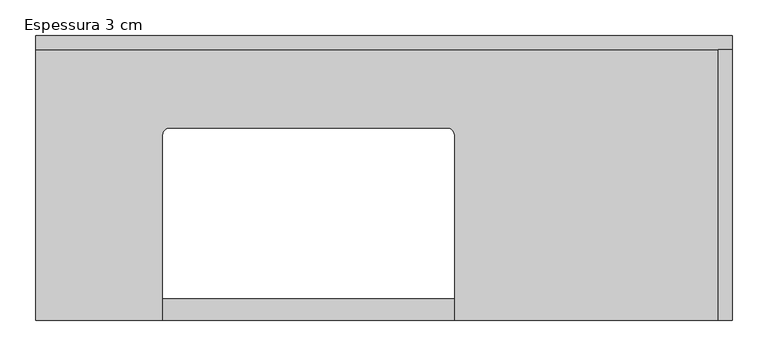
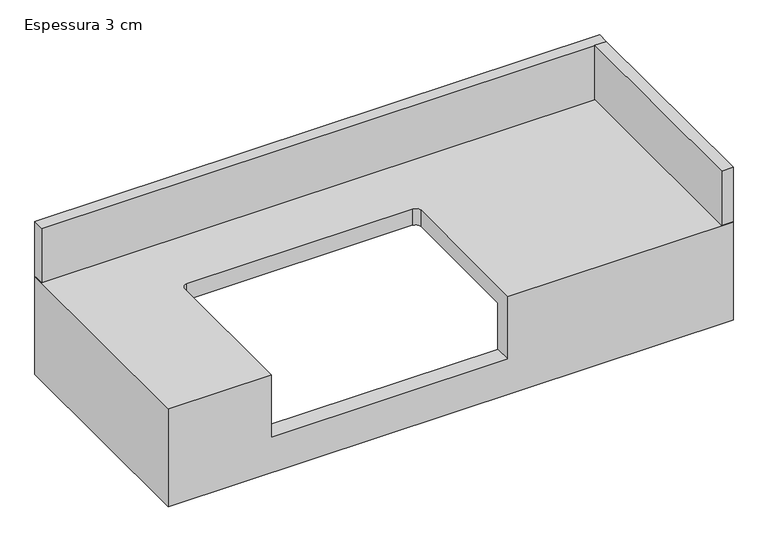
"""IFC4 building model written with IfcOpenShell, lengths in millimetres: furniture geometry, CC_BANCADA BANHEIRO COM CUBA_CANTO RETO : Espessura 3 cm."""

from ifc_helpers import new_model, si_unit, frame, origin, place, context, project, spatial, polyline, circle_curve, outline, extrude, source, transform, mapped, element, save
from ifc_brep_helpers import plane_surface, revolved_surface, advanced_brep


def espessura_3_cm_7a2f0677(model_context):
    return source(origin(), model_context, "Body", "SolidModel", [
        advanced_brep(
        [(750.0, 300.0, 860.0), (-228.0, 300.0, 860.0), (-228.0, -100.0, 860.0), (-50.0, -100.0, 860.0), (-50.0, 160.0, 860.0), (-40.0, 170.0, 860.0), (350.0, 170.0, 860.0), (360.0, 160.0, 860.0), (360.0, -100.0, 860.0), (750.0, -100.0, 860.0), (750.0, 300.0, 680.0), (720.0, 300.0, 680.0), (720.0, 300.0, 830.0), (-198.0, 300.0, 830.0), (-198.0, 300.0, 680.0), (-228.0, 300.0, 680.0), (-228.0, -100.0, 680.0), (750.0, -100.0, 680.0), (360.0, -100.0, 745.0), (-50.0, -100.0, 745.0), (720.0, -70.0, 830.0), (360.0, -70.0, 830.0), (360.0, 160.0, 830.0), (350.0, 170.0, 830.0), (-40.0, 170.0, 830.0), (-50.0, 160.0, 830.0), (-50.0, -70.0, 830.0), (-198.0, -70.0, 830.0), (-198.0, -70.0, 680.0), (-50.0, -70.0, 745.0), (360.0, -70.0, 745.0), (720.0, -70.0, 680.0)],
        [
            (0, 1),
            (1, 2),
            (2, 3),
            (3, 4),
            (4, 5, circle_curve(frame((-40.0, 160.0, 860.0), z_axis=(0.0, 0.0, -1.0), x_axis=(0.0, 1.0, 0.0)), 10.0)),
            (5, 6),
            (6, 7, circle_curve(frame((350.0, 160.0, 860.0), z_axis=(0.0, 0.0, -1.0), x_axis=(0.0, 1.0, 0.0)), 10.0)),
            (7, 8),
            (8, 9),
            (9, 0),
            (0, 10),
            (10, 11),
            (11, 12),
            (12, 13),
            (13, 14),
            (14, 15),
            (15, 1),
            (15, 16),
            (16, 2),
            (16, 17),
            (17, 9),
            (8, 18),
            (18, 19),
            (19, 3),
            (17, 10),
            (12, 20),
            (20, 21),
            (21, 22),
            (22, 23, circle_curve(frame((350.0, 160.0, 830.0), z_axis=(0.0, 0.0, 1.0), x_axis=(0.0, 1.0, 0.0)), 10.0)),
            (23, 24),
            (24, 25, circle_curve(frame((-40.0, 160.0, 830.0), z_axis=(0.0, 0.0, 1.0), x_axis=(0.0, 1.0, 0.0)), 10.0)),
            (25, 26),
            (26, 27),
            (27, 13),
            (27, 28),
            (28, 14),
            (26, 29),
            (29, 30),
            (30, 21),
            (20, 31),
            (31, 28),
            (11, 31),
            (5, 24),
            (23, 6),
            (18, 30),
            (29, 19),
            (4, 25),
            (7, 22),
        ],
        [
            plane_surface(frame((-228.0, 300.0, 860.0), z_axis=(0.0, 0.0, 1.0), x_axis=(-1.0, 0.0, 0.0))),
            plane_surface(frame((750.0, 300.0, 860.0), z_axis=(0.0, 1.0, 0.0), x_axis=(0.0, 0.0, -1.0))),
            plane_surface(frame((-228.0, 300.0, 860.0), z_axis=(-1.0, 0.0, 0.0), x_axis=(0.0, 0.0, -1.0))),
            plane_surface(frame((-228.0, -100.0, 860.0), z_axis=(0.0, -1.0, 0.0), x_axis=(0.0, 0.0, -1.0))),
            plane_surface(frame((750.0, -100.0, 860.0), z_axis=(1.0, 0.0, 0.0), x_axis=(0.0, 0.0, -1.0))),
            plane_surface(frame((-198.0, 300.0, 830.0), z_axis=(0.0, 0.0, -1.0), x_axis=(-1.0, 0.0, 0.0))),
            plane_surface(frame((-198.0, 300.0, 830.0), z_axis=(1.0, 0.0, 0.0), x_axis=(0.0, 0.0, -1.0))),
            plane_surface(frame((-198.0, -70.0, 830.0), z_axis=(0.0, 1.0, 0.0), x_axis=(0.0, 0.0, -1.0))),
            plane_surface(frame((720.0, -70.0, 830.0), z_axis=(-1.0, 0.0, 0.0), x_axis=(0.0, 0.0, -1.0))),
            plane_surface(frame((750.0, -100.0, 680.0), z_axis=(0.0, 0.0, -1.0), x_axis=(0.0, 1.0, 0.0))),
            plane_surface(frame((-40.0, 170.0, 745.0), z_axis=(0.0, -1.0, 0.0), x_axis=(0.0, 0.0, 1.0))),
            plane_surface(frame((350.0, 170.0, 745.0), z_axis=(0.0, 0.0, 1.0), x_axis=(1.0, 0.0, 0.0))),
            revolved_surface(polyline([(-40.0, 170.0, 830.0), (-40.0, 170.0, 860.0)]), (-40.0, 160.0, 900.0), (0.0, 0.0, -1.0)),
            plane_surface(frame((-50.0, -230.0, 745.0), z_axis=(1.0, 0.0, 0.0), x_axis=(0.0, 0.0, 1.0))),
            plane_surface(frame((360.0, 160.0, 745.0), z_axis=(-1.0, 0.0, 0.0), x_axis=(0.0, 0.0, 1.0))),
            revolved_surface(polyline([(350.0, 170.0, 830.0), (350.0, 170.0, 860.0)]), (350.0, 160.0, 900.0), (0.0, 0.0, -1.0)),
        ],
        [
            (0, [[1, 2, 3, 4, 5, 6, 7, 8, 9, 10]]),
            (1, [[-1, 11, 12, 13, 14, 15, 16, 17]]),
            (2, [[-2, -17, 18, 19]]),
            (3, [[-3, -19, 20, 21, -9, 22, 23, 24]]),
            (4, [[-10, -21, 25, -11]]),
            (5, [[26, 27, 28, 29, 30, 31, 32, 33, 34, -14]]),
            (6, [[-34, 35, 36, -15]]),
            (7, [[-33, 37, 38, 39, -27, 40, 41, -35]]),
            (8, [[-26, -13, 42, -40]]),
            (9, [[-12, -25, -20, -18, -16, -36, -41, -42]]),
            (10, [[-6, 43, -30, 44]]),
            (11, [[-23, 45, -38, 46]]),
            (12, [[-5, 47, -31, -43]]),
            (13, [[-4, -24, -46, -37, -32, -47]]),
            (14, [[-8, 48, -28, -39, -45, -22]]),
            (15, [[-7, -44, -29, -48]]),
        ],
    ),
        extrude(outline(polyline([(730.0, 280.0), (750.0, 280.0), (750.0, -100.0), (730.0, -100.0), (730.0, 280.0)])), frame((0.0, 0.0, 860.0), z_axis=(0.0, 0.0, 1.0), x_axis=(1.0, 0.0, 0.0)), (0.0, 0.0, 1.0), 100.0),
        extrude(outline(polyline([(750.0, 300.0), (750.0, 280.0), (-228.0, 280.0), (-228.0, 300.0), (750.0, 300.0)])), frame((0.0, 0.0, 860.0), z_axis=(0.0, 0.0, 1.0), x_axis=(1.0, 0.0, 0.0)), (0.0, 0.0, 1.0), 100.0),
    ])


if __name__ == "__main__":
    model = new_model("IFC4")
    model_context = context("Model", 3, world=origin())
    ifc_project = project(units=[si_unit("LENGTHUNIT", "METRE", prefix="MILLI")], contexts=[model_context])
    site = spatial("IfcSite", under=ifc_project)
    building = spatial("IfcBuilding", under=site)
    placement = place(None, origin())
    espessura_3_cm_shape = espessura_3_cm_7a2f0677(model_context)
    element("IfcFurniture", 1, ObjectType="CC_BANCADA BANHEIRO COM CUBA_CANTO RETO : Espessura 3 cm", at=placement, inside=building, context=model_context, shape_type="MappedRepresentation", body=[
        mapped(espessura_3_cm_shape, transform((0.0, 0.0, 0.0), x_axis=(1.0, 0.0, 0.0), y_axis=(0.0, 1.0, 0.0), z_axis=(0.0, 0.0, 1.0))),
    ])
    save(model, "model.ifc")

# Revit data of these elements
# Type "CC_BANCADA BANHEIRO COM CUBA_CANTO RETO : Espessura 3 cm"
#   Uso HS [instance default] = ""
#   h TESTEIRA AUX [instance default] = 0.15 m
#   Altura testeira [instance default] = 0.15 m
#   Altura rodapia [instance default] = 0.10 m
#   Espessura rodapia [instance default] = 0.02 m
#   Prof/2 [instance default] = 0.20 m
#   Offset cuba esquerda [instance default] = 0.40 m
#   Depth [instance default] = 1.20 m
#   Width [instance default] = 0.40 m
#   Espessura bancada = 0.03 m
#   Comprimento [instance default] = 1.20 m
#   Height [instance default] = 0.86 m
#   Testeira [instance default] = yes
#   Rodapia fundo [instance default] = no
#   Rodapia esquerda [instance default] = no
#   Rodapia direita [instance default] = no
#   Material porta-toalha [instance default] = .CROMADO
#   Material hidráulico [instance default] = .CROMADO
#   Material cuba [instance default] = .PORCELANA BRANCA
#   Material bancada [instance default] = .GRANITO_BRANCO_ITAUNAS
#   Assembly Code = ""
# Element 1 (IfcFurniture, "CC_BANCADA BANHEIRO COM CUBA_CANTO RETO : Espessura 3 cm")
#   Uso HS = "BANHO SUÍTE 3"
#   Offset cuba esquerda = 0.178 m
#   Depth = 0.978 m
#   Comprimento = 0.978 m
#   Rodapia fundo = yes
#   Rodapia direita = yes
#   Materials on its faces: ".GRANITO_BRANCO_ITAUNAS"
# Materials
#   ".CROMADO": class "CC_METAIS", colour RGB 211 223 226, transparency 0, Cost = 0
#   ".PORCELANA BRANCA": class "CC_PORCELANA", colour RGB 230 230 230, transparency 0, Cost = 0
#   ".GRANITO_BRANCO_ITAUNAS": class ".CC_PEDRA REVEST.", colour RGB 202 195 174, transparency 0, Description = "Revestimento em granito", Cost = 0
